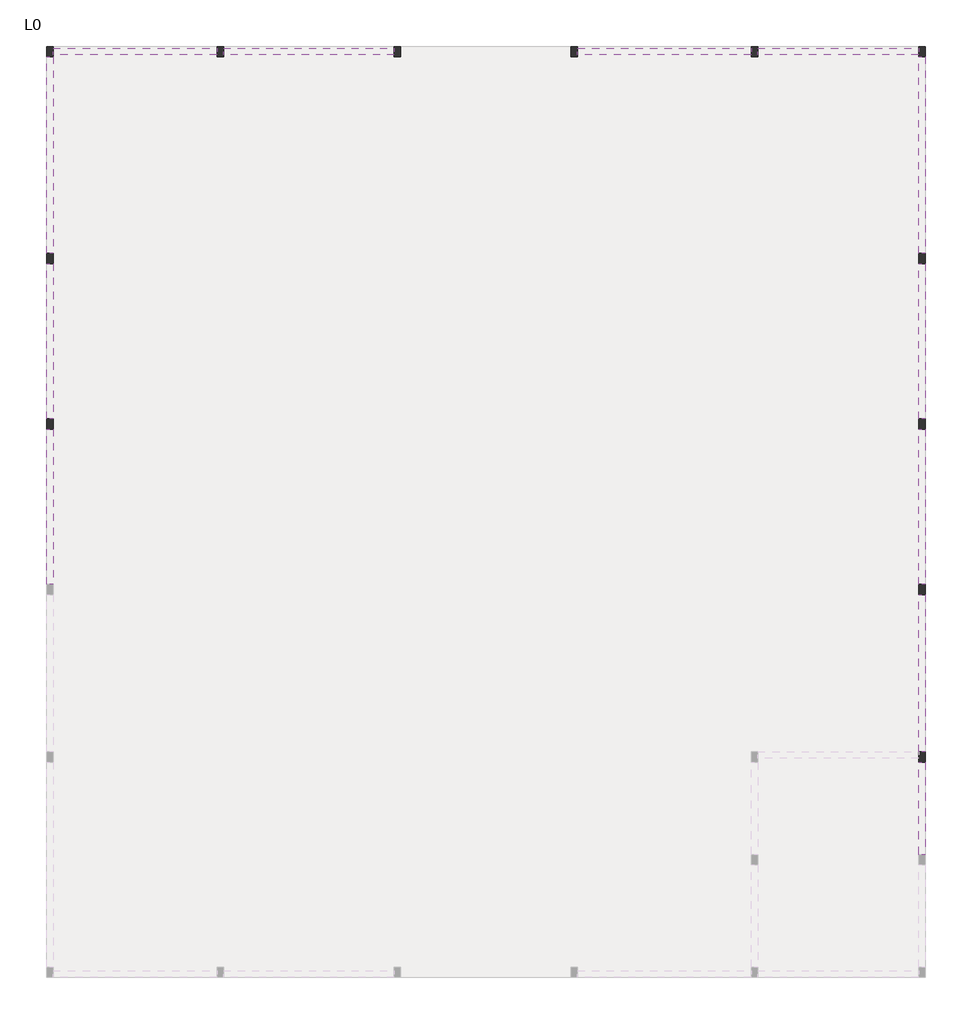
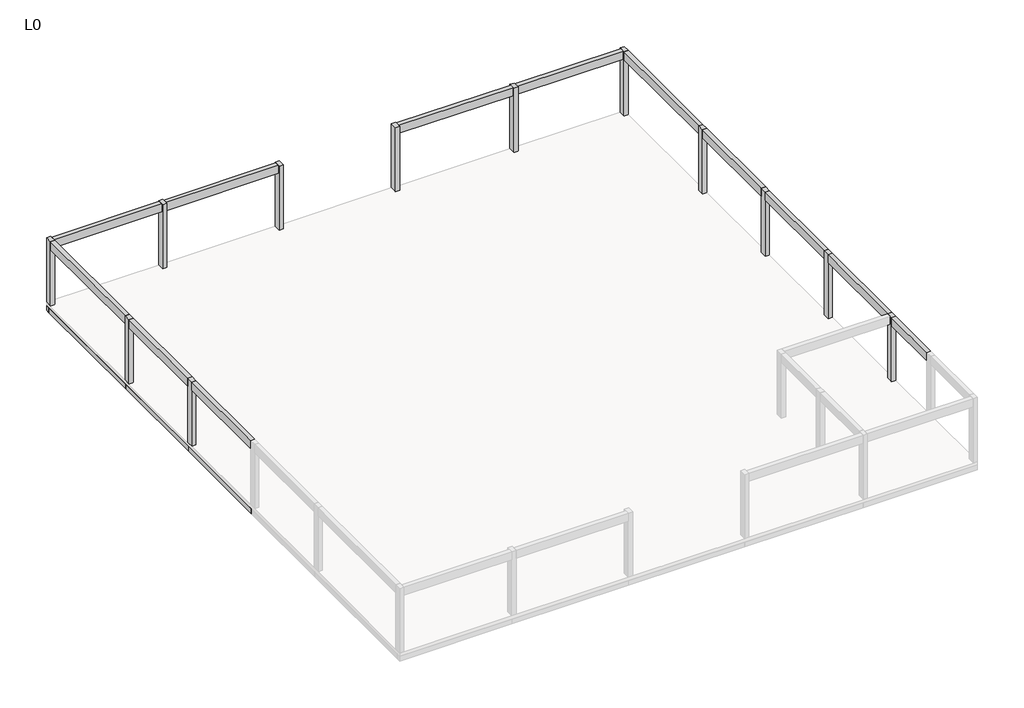
# One storey, part 2 of 2: 37 beams, 12 columns.
"""IFC4 building model written with IfcOpenShell, lengths in millimetres."""

import ifcopenshell
import ifcopenshell.guid

model = None  # the IFC model being written
_history = None  # IfcOwnerHistory: only IFC2X3 demands one
_inside = {}  # id of a spatial element -> (the spatial element, [elements in it])
_under = {}  # id of a project, library or spatial element -> (it, [spatial elements below it])
_declared = {}  # id of a project -> (the project, [libraries it declares])
_typed = {}  # id of a type object -> (the type object, [elements of that type])
_made_of = {}  # id of a material, layer set ... -> (it, [elements and type objects made of it])


def new_model(schema):
    """Start an empty IFC model of exactly this schema.

    Asked for "IFC4X3", IfcOpenShell would pick the latest addendum, in which some entities
    have other attributes; the version numbers below select the first issue.
    IFC2X3 requires an IfcOwnerHistory on every rooted entity: one is made here for all.
    """
    global model, _history
    if schema == "IFC4X3":
        model = ifcopenshell.file(schema_version=(4, 3, 0, 0))
    else:
        model = ifcopenshell.file(schema=schema)
    _inside.clear()
    _under.clear()
    _declared.clear()
    _typed.clear()
    _made_of.clear()
    _history = None
    if model.schema == "IFC2X3":
        org = make("IfcOrganization", Name="unknown")
        user = make(
            "IfcPersonAndOrganization",
            ThePerson=make("IfcPerson", FamilyName="unknown"),
            TheOrganization=org,
        )
        app = make(
            "IfcApplication",
            ApplicationDeveloper=org,
            Version="unknown",
            ApplicationFullName="unknown",
            ApplicationIdentifier="unknown",
        )
        _history = make(
            "IfcOwnerHistory",
            OwningUser=user,
            OwningApplication=app,
            ChangeAction="ADDED",
            CreationDate=0,
        )
    return model


def make(cls, **values):
    """One entity of the class cls with the attributes given. An attribute that is None is left unset."""
    return model.create_entity(
        cls, **{name: value for name, value in values.items() if value is not None}
    )


def rooted(cls, **values):
    """An entity with a GlobalId (a new one), such as an element, a storey or a relation."""
    return make(cls, GlobalId=ifcopenshell.guid.new(), OwnerHistory=_history, **values)


def si_unit(unit_type, name, prefix=None):
    """IfcSIUnit, for example si_unit("LENGTHUNIT", "METRE", prefix="MILLI")."""
    return make("IfcSIUnit", UnitType=unit_type, Prefix=prefix, Name=name)


def assignment(units):
    """IfcUnitAssignment: the units of a project."""
    return None if units is None else make("IfcUnitAssignment", Units=units)


def point(xyz):
    """IfcCartesianPoint."""
    return None if xyz is None else make("IfcCartesianPoint", Coordinates=xyz)


def direction(xyz):
    """IfcDirection."""
    return None if xyz is None else make("IfcDirection", DirectionRatios=xyz)


def frame(location, z_axis=None, x_axis=None):
    """IfcAxis2Placement3D, a coordinate frame: its origin and axes. An axis left out is left unset."""
    return make(
        "IfcAxis2Placement3D",
        Location=point(location),
        Axis=direction(z_axis),
        RefDirection=direction(x_axis),
    )


def origin():
    """The frame at (0, 0, 0) with its axes left unset."""
    return frame((0.0, 0.0, 0.0))


def origin_with_axes():
    """The frame at (0, 0, 0) with the z axis (0, 0, 1) and the x axis (1, 0, 0) written out."""
    return frame((0.0, 0.0, 0.0), z_axis=(0.0, 0.0, 1.0), x_axis=(1.0, 0.0, 0.0))


def place(relative_to, where):
    """IfcLocalPlacement: puts the frame where relative to a parent placement (None: the world)."""
    return make(
        "IfcLocalPlacement", PlacementRelTo=relative_to, RelativePlacement=where
    )


def context(
    kind, dimensions, precision=None, world=None, true_north=None, identifier=None
):
    """IfcGeometricRepresentationContext, for example the 3D "Model" context."""
    return make(
        "IfcGeometricRepresentationContext",
        ContextIdentifier=identifier,
        ContextType=kind,
        CoordinateSpaceDimension=dimensions,
        Precision=precision,
        WorldCoordinateSystem=world,
        TrueNorth=true_north,
    )


def project(units=None, contexts=None):
    """IfcProject with its units and contexts."""
    return rooted(
        "IfcProject",
        Name="project",
        RepresentationContexts=contexts,
        UnitsInContext=assignment(units),
    )


def spatial(cls, under=None, at=None, **own):
    """A site, building, storey or space (cls), placed at a placement, below another one or the project."""
    s = rooted(cls, ObjectPlacement=at, **own)
    if under is not None:
        _under.setdefault(under.id(), (under, []))[1].append(s)
    return s


def polyline(points):
    """IfcPolyline through the points."""
    return make("IfcPolyline", Points=[point(p) for p in points])


def outline(outer, holes=None, kind="AREA"):
    """IfcArbitraryClosedProfileDef: a profile drawn as a closed curve; with holes, ...WithVoids."""
    if holes is None:
        return make("IfcArbitraryClosedProfileDef", ProfileType=kind, OuterCurve=outer)
    return make(
        "IfcArbitraryProfileDefWithVoids",
        ProfileType=kind,
        OuterCurve=outer,
        InnerCurves=holes,
    )


def extrude(swept, where, along, depth):
    """IfcExtrudedAreaSolid: the profile swept, set in the frame where, extruded along a direction by depth."""
    return make(
        "IfcExtrudedAreaSolid",
        SweptArea=swept,
        Position=where,
        ExtrudedDirection=direction(along),
        Depth=depth,
    )


def faces_of(points, faces, orient=None, outer=None):
    """IfcFace entities. A face is a list of loops; a loop is a list of indices into points, from 0.

    orient and outer hold one flag for each loop. By default every Orientation is true, the
    first loop of a face is its IfcFaceOuterBound and the others are IfcFaceBound.
    """
    made = []
    for i, loops in enumerate(faces):
        bounds = []
        for j, loop in enumerate(loops):
            is_outer = j == 0 if outer is None else outer[i][j]
            bounds.append(
                make(
                    "IfcFaceOuterBound" if is_outer else "IfcFaceBound",
                    Bound=make("IfcPolyLoop", Polygon=[points[k] for k in loop]),
                    Orientation=True if orient is None else orient[i][j],
                )
            )
        made.append(make("IfcFace", Bounds=bounds))
    return made


def faceted_brep(points, faces, orient=None, outer=None, voids=None):
    """IfcFacetedBrep: a solid bounded by flat faces; with voids (closed shells), ...WithVoids."""
    shared = [point(p) for p in points]
    hull = make("IfcClosedShell", CfsFaces=faces_of(shared, faces, orient, outer))
    if voids is None:
        return make("IfcFacetedBrep", Outer=hull)
    return make(
        "IfcFacetedBrepWithVoids",
        Outer=hull,
        Voids=[
            make(cls, CfsFaces=faces_of(shared, fs, o, b)) for cls, fs, o, b in voids
        ],
    )


def shape(context_of_items, identifier, shape_type, items):
    """IfcShapeRepresentation: the items that make up one representation, for example the "Body"."""
    return make(
        "IfcShapeRepresentation",
        ContextOfItems=context_of_items,
        RepresentationIdentifier=identifier,
        RepresentationType=shape_type,
        Items=items,
    )


def made_of(thing, what):
    """Note that an element or type object is made of a material, layer set ...; save() writes the relation."""
    if what is not None:
        _made_of.setdefault(what.id(), (what, []))[1].append(thing)
    return thing


def element(
    cls,
    number,
    at=None,
    inside=None,
    cuts=None,
    type_object=None,
    material=None,
    context=None,
    identifier="Body",
    shape_type=None,
    held_by="IfcProductDefinitionShape",
    body=None,
    shapes=None,
    **own,
):
    """One element of the class cls, such as IfcWall. Its Tag is "e" and its number.

    at: its placement. inside: the storey or other place that contains it. cuts: it is an
    opening in that element (IfcRelVoidsElement). A single representation is given by context,
    identifier, shape_type and body (its items); several are given by shapes. held_by: the class
    of the entity that holds the representations. save() writes the other relations.
    """
    e = rooted(cls, Tag="e%d" % number, ObjectPlacement=at, **own)
    if body is not None:
        shapes = [shape(context, identifier, shape_type, body)]
    if shapes is not None:
        e.Representation = make(held_by, Representations=shapes)
    if inside is not None:
        _inside.setdefault(inside.id(), (inside, []))[1].append(e)
    if cuts is not None:
        rooted(
            "IfcRelVoidsElement", RelatingBuildingElement=cuts, RelatedOpeningElement=e
        )
    if type_object is not None:
        _typed.setdefault(type_object.id(), (type_object, []))[1].append(e)
    return made_of(e, material)


def aggregate(whole, parts):
    """IfcRelAggregates: a whole, such as a stair, and the parts it consists of."""
    return rooted("IfcRelAggregates", RelatingObject=whole, RelatedObjects=parts)


def save(model, path):
    """Write the relations noted so far, then the file.

    IfcRelAggregates (storeys below a building ...), IfcRelContainedInSpatialStructure (elements
    in a storey), IfcRelDefinesByType, IfcRelAssociatesMaterial and IfcRelDeclares: one each for
    every whole, place, type object, material and project.
    """
    for whole, parts in _under.values():
        aggregate(whole, parts)
    for where, things in _inside.values():
        rooted(
            "IfcRelContainedInSpatialStructure",
            RelatedElements=things,
            RelatingStructure=where,
        )
    for kind, things in _typed.values():
        rooted("IfcRelDefinesByType", RelatedObjects=things, RelatingType=kind)
    for what, things in _made_of.values():
        rooted("IfcRelAssociatesMaterial", RelatedObjects=things, RelatingMaterial=what)
    for by, libraries in _declared.values():
        rooted("IfcRelDeclares", RelatingContext=by, RelatedDefinitions=libraries)
    model.write(path)


model = new_model("IFC4")

# Units and contexts
model_context = context("Model", 3, world=origin())
ifc_project = project(units=[si_unit("LENGTHUNIT", "METRE", prefix="MILLI")], contexts=[model_context])

# Site, building, storey
site = spatial("IfcSite", under=ifc_project)
building = spatial("IfcBuilding", under=site)
storey = spatial("IfcBuildingStorey", under=building, Name="L0", Elevation=0.0)

# Beams
placement = place(None, origin())
element("IfcBeam", 1, ObjectType="Concrete-Rectangular Beam : 25 x 50", at=placement, inside=storey, context=model_context, shape_type="Brep", body=[
    faceted_brep([(17000.0, 18000.0, -500.0), (10270.0, 18000.0, -500.0), (10270.0, 18000.0, -200.0), (17000.0, 18000.0, -200.0), (10270.0, 17750.0, -500.0), (17000.0, 17750.0, -500.0), (16750.0, 17750.0, -500.0), (10520.0, 17750.0, -500.0), (17000.0, 17750.0, -200.0), (16750.0, 17750.0, -200.0), (10520.0, 17750.0, -200.0), (10270.0, 17750.0, -200.0)], [[[0, 1, 2, 3]], [[4, 1, 0, 5, 6, 7]], [[4, 7, 6, 5, 8, 9, 10, 11]], [[1, 4, 11, 2]], [[5, 0, 3, 8]], [[3, 2, 11, 10, 9, 8]]]),
])
element("IfcBeam", 2, ObjectType="Concrete-Rectangular Beam : 25 x 50", at=placement, inside=storey, context=model_context, shape_type="Brep", body=[
    faceted_brep([(10270.0, 18000.0, -500.0), (3300.0, 18000.0, -500.0), (3300.0, 18000.0, -200.0), (10270.0, 18000.0, -200.0), (3300.0, 17750.0, -500.0), (10270.0, 17750.0, -500.0), (3550.0, 17750.0, -500.0), (10270.0, 17750.0, -200.0), (3550.0, 17750.0, -200.0), (3300.0, 17750.0, -200.0)], [[[0, 1, 2, 3]], [[4, 1, 0, 5, 6]], [[4, 6, 5, 7, 8, 9]], [[1, 4, 9, 2]], [[5, 0, 3, 7]], [[3, 2, 9, 8, 7]]]),
])
element("IfcBeam", 3, ObjectType="Concrete-Rectangular Beam : 25 x 50", at=placement, inside=storey, context=model_context, shape_type="Brep", body=[
    faceted_brep([(3300.0, 18000.0, -500.0), (-3550.0, 18000.0, -500.0), (-3550.0, 18000.0, -200.0), (3300.0, 18000.0, -200.0), (-3550.0, 17750.0, -500.0), (3300.0, 17750.0, -500.0), (-3300.0, 17750.0, -500.0), (3300.0, 17750.0, -200.0), (-3300.0, 17750.0, -200.0), (-3550.0, 17750.0, -200.0)], [[[0, 1, 2, 3]], [[4, 1, 0, 5, 6]], [[4, 6, 5, 7, 8, 9]], [[1, 4, 9, 2]], [[5, 0, 3, 7]], [[3, 2, 9, 8, 7]]]),
])
element("IfcBeam", 4, ObjectType="Concrete-Rectangular Beam : 25 x 50", at=placement, inside=storey, context=model_context, shape_type="Brep", body=[
    faceted_brep([(-3550.0, 18000.0, -500.0), (-10400.0, 18000.0, -500.0), (-10400.0, 18000.0, -200.0), (-3550.0, 18000.0, -200.0), (-10400.0, 17750.0, -500.0), (-3550.0, 17750.0, -500.0), (-10150.0, 17750.0, -500.0), (-3550.0, 17750.0, -200.0), (-10150.0, 17750.0, -200.0), (-10400.0, 17750.0, -200.0)], [[[0, 1, 2, 3]], [[4, 1, 0, 5, 6]], [[4, 6, 5, 7, 8, 9]], [[1, 4, 9, 2]], [[5, 0, 3, 7]], [[3, 2, 9, 8, 7]]]),
])
element("IfcBeam", 5, ObjectType="Concrete-Rectangular Beam : 25 x 50", at=placement, inside=storey, context=model_context, shape_type="Brep", body=[
    faceted_brep([(-10400.0, 18000.0, -500.0), (-17000.0, 18000.0, -500.0), (-17000.0, 18000.0, -200.0), (-10400.0, 18000.0, -200.0), (-17000.0, 17750.0, -500.0), (-10400.0, 17750.0, -500.0), (-16750.0, 17750.0, -500.0), (-10400.0, 17750.0, -200.0), (-16750.0, 17750.0, -200.0), (-17000.0, 17750.0, -200.0)], [[[0, 1, 2, 3]], [[4, 1, 0, 5, 6]], [[4, 6, 5, 7, 8, 9]], [[1, 4, 9, 2]], [[5, 0, 3, 7]], [[3, 2, 9, 8, 7]]]),
])
element("IfcBeam", 6, ObjectType="Concrete-Rectangular Beam : 25 x 50", at=placement, inside=storey, context=model_context, shape_type="Brep", body=[
    faceted_brep([(17000.0, 9925.0, -500.0), (16750.0, 9925.0, -500.0), (10520.0, 9925.0, -500.0), (10520.0, 9925.0, -200.0), (16750.0, 9925.0, -200.0), (17000.0, 9925.0, -200.0), (17000.0, 9675.0, -500.0), (16750.0, 9675.0, -500.0), (10520.0, 9675.0, -500.0), (17000.0, 9675.0, -200.0), (16750.0, 9675.0, -200.0), (10520.0, 9675.0, -200.0)], [[[0, 1, 2, 3, 4, 5]], [[0, 6, 7, 8, 2, 1]], [[8, 7, 6, 9, 10, 11]], [[6, 0, 5, 9]], [[2, 8, 11, 3]], [[5, 4, 3, 11, 10, 9]]]),
])
element("IfcBeam", 7, ObjectType="Concrete-Rectangular Beam : 25 x 50", at=placement, inside=storey, context=model_context, shape_type="Brep", body=[
    faceted_brep([(17000.0, 3525.0, -500.0), (16750.0, 3525.0, -500.0), (10520.0, 3525.0, -500.0), (10270.0, 3525.0, -500.0), (3550.0, 3525.0, -500.0), (3300.0, 3525.0, -500.0), (-3300.0, 3525.0, -500.0), (-3550.0, 3525.0, -500.0), (-10150.0, 3525.0, -500.0), (-10150.0, 3525.0, -200.0), (-3550.0, 3525.0, -200.0), (-3300.0, 3525.0, -200.0), (3300.0, 3525.0, -200.0), (3550.0, 3525.0, -200.0), (10270.0, 3525.0, -200.0), (10520.0, 3525.0, -200.0), (16750.0, 3525.0, -200.0), (17000.0, 3525.0, -200.0), (17000.0, 3275.0, -500.0), (16750.0, 3275.0, -500.0), (10520.0, 3275.0, -500.0), (10270.0, 3275.0, -500.0), (3550.0, 3275.0, -500.0), (3300.0, 3275.0, -500.0), (-3300.0, 3275.0, -500.0), (-3550.0, 3275.0, -500.0), (-10150.0, 3275.0, -500.0), (17000.0, 3275.0, -200.0), (16750.0, 3275.0, -200.0), (10520.0, 3275.0, -200.0), (10270.0, 3275.0, -200.0), (3550.0, 3275.0, -200.0), (3300.0, 3275.0, -200.0), (-3300.0, 3275.0, -200.0), (-3550.0, 3275.0, -200.0), (-10150.0, 3275.0, -200.0)], [[[0, 1, 2, 3, 4, 5, 6, 7, 8, 9, 10, 11, 12, 13, 14, 15, 16, 17]], [[0, 18, 19, 20, 21, 22, 23, 24, 25, 26, 8, 7, 6, 5, 4, 3, 2, 1]], [[26, 25, 24, 23, 22, 21, 20, 19, 18, 27, 28, 29, 30, 31, 32, 33, 34, 35]], [[18, 0, 17, 27]], [[8, 26, 35, 9]], [[17, 16, 15, 14, 13, 12, 11, 10, 9, 35, 34, 33, 32, 31, 30, 29, 28, 27]]]),
])
element("IfcBeam", 8, ObjectType="Concrete-Rectangular Beam : 25 x 50", at=placement, inside=storey, context=model_context, shape_type="Brep", body=[
    faceted_brep([(-16750.0, -2875.0, -500.0), (-16750.0, 3275.0, -500.0), (-16750.0, 3525.0, -500.0), (-16750.0, 3525.0, -200.0), (-16750.0, 3275.0, -200.0), (-16750.0, -2875.0, -200.0), (-17000.0, 3525.0, -500.0), (-17000.0, -2875.0, -500.0), (-17000.0, -2875.0, -200.0), (-17000.0, 3525.0, -200.0)], [[[0, 1, 2, 3, 4, 5]], [[6, 2, 1, 0, 7]], [[6, 7, 8, 9]], [[2, 6, 9, 3]], [[7, 0, 5, 8]], [[5, 4, 3, 9, 8]]]),
])
element("IfcBeam", 9, ObjectType="Concrete-Rectangular Beam : 25 x 50", at=placement, inside=storey, context=model_context, shape_type="Brep", body=[
    faceted_brep([(-16750.0, 3525.0, -500.0), (-16750.0, 9675.0, -500.0), (-16750.0, 9925.0, -500.0), (-16750.0, 9925.0, -200.0), (-16750.0, 9675.0, -200.0), (-16750.0, 3525.0, -200.0), (-17000.0, 9925.0, -500.0), (-17000.0, 3525.0, -500.0), (-17000.0, 3525.0, -200.0), (-17000.0, 9925.0, -200.0)], [[[0, 1, 2, 3, 4, 5]], [[6, 2, 1, 0, 7]], [[6, 7, 8, 9]], [[2, 6, 9, 3]], [[7, 0, 5, 8]], [[5, 4, 3, 9, 8]]]),
])
element("IfcBeam", 10, ObjectType="Concrete-Rectangular Beam : 25 x 50", at=placement, inside=storey, context=model_context, shape_type="SweptSolid", body=[
    extrude(outline(polyline([(-17000.0, 17750.0), (-16750.0, 17750.0), (-16750.0, 9925.0), (-17000.0, 9925.0), (-17000.0, 17750.0)])), frame((0.0, 0.0, -500.0), z_axis=(0.0, 0.0, 1.0), x_axis=(1.0, 0.0, 0.0)), (0.0, 0.0, 1.0), 300.0),
])
element("IfcBeam", 11, ObjectType="Concrete-Rectangular Beam : 25 x 50", at=placement, inside=storey, context=model_context, shape_type="SweptSolid", body=[
    extrude(outline(polyline([(17000.0, -13448.5675387), (16750.0, -13448.5675387), (16750.0, -9595.0), (17000.0, -9595.0), (17000.0, -13448.5675387)])), frame((0.0, 0.0, -500.0), z_axis=(0.0, 0.0, 1.0), x_axis=(1.0, 0.0, 0.0)), (0.0, 0.0, 1.0), 300.0),
])
element("IfcBeam", 12, ObjectType="Concrete-Rectangular Beam : 25 x 50", at=placement, inside=storey, context=model_context, shape_type="SweptSolid", body=[
    extrude(outline(polyline([(16750.0, -3125.0), (17000.0, -3125.0), (17000.0, -9345.0), (16750.0, -9345.0), (16750.0, -3125.0)])), frame((0.0, 0.0, -500.0), z_axis=(0.0, 0.0, 1.0), x_axis=(1.0, 0.0, 0.0)), (0.0, 0.0, 1.0), 300.0),
])
element("IfcBeam", 13, ObjectType="Concrete-Rectangular Beam : 25 x 50", at=placement, inside=storey, context=model_context, shape_type="SweptSolid", body=[
    extrude(outline(polyline([(16750.0, 3275.0), (17000.0, 3275.0), (17000.0, -2875.0), (16750.0, -2875.0), (16750.0, 3275.0)])), frame((0.0, 0.0, -500.0), z_axis=(0.0, 0.0, 1.0), x_axis=(1.0, 0.0, 0.0)), (0.0, 0.0, 1.0), 300.0),
])
element("IfcBeam", 14, ObjectType="Concrete-Rectangular Beam : 25 x 50", at=placement, inside=storey, context=model_context, shape_type="SweptSolid", body=[
    extrude(outline(polyline([(16750.0, 9675.0), (17000.0, 9675.0), (17000.0, 3525.0), (16750.0, 3525.0), (16750.0, 9675.0)])), frame((0.0, 0.0, -500.0), z_axis=(0.0, 0.0, 1.0), x_axis=(1.0, 0.0, 0.0)), (0.0, 0.0, 1.0), 300.0),
])
element("IfcBeam", 15, ObjectType="Concrete-Rectangular Beam : 25 x 50", at=placement, inside=storey, context=model_context, shape_type="SweptSolid", body=[
    extrude(outline(polyline([(17000.0, 9925.0), (16750.0, 9925.0), (16750.0, 17750.0), (17000.0, 17750.0), (17000.0, 9925.0)])), frame((0.0, 0.0, -500.0), z_axis=(0.0, 0.0, 1.0), x_axis=(1.0, 0.0, 0.0)), (0.0, 0.0, 1.0), 300.0),
])
element("IfcBeam", 16, ObjectType="Concrete-Rectangular Beam : 25 x 50", at=placement, inside=storey, context=model_context, shape_type="SweptSolid", body=[
    extrude(outline(polyline([(-10400.0, 17750.0), (-10150.0, 17750.0), (-10150.0, 9925.0), (-10400.0, 9925.0), (-10400.0, 17750.0)])), frame((0.0, 0.0, -500.0), z_axis=(0.0, 0.0, 1.0), x_axis=(1.0, 0.0, 0.0)), (0.0, 0.0, 1.0), 300.0),
])
element("IfcBeam", 17, ObjectType="Concrete-Rectangular Beam : 25 x 50", at=placement, inside=storey, context=model_context, shape_type="SweptSolid", body=[
    extrude(outline(polyline([(-3550.0, 17750.0), (-3300.0, 17750.0), (-3300.0, 9925.0), (-3550.0, 9925.0), (-3550.0, 17750.0)])), frame((0.0, 0.0, -500.0), z_axis=(0.0, 0.0, 1.0), x_axis=(1.0, 0.0, 0.0)), (0.0, 0.0, 1.0), 300.0),
])
element("IfcBeam", 18, ObjectType="Concrete-Rectangular Beam : 25 x 50", at=placement, inside=storey, context=model_context, shape_type="SweptSolid", body=[
    extrude(outline(polyline([(3300.0, 17750.0), (3550.0, 17750.0), (3550.0, 9925.0), (3300.0, 9925.0), (3300.0, 17750.0)])), frame((0.0, 0.0, -500.0), z_axis=(0.0, 0.0, 1.0), x_axis=(1.0, 0.0, 0.0)), (0.0, 0.0, 1.0), 300.0),
])
element("IfcBeam", 19, ObjectType="Concrete-Rectangular Beam : 25 x 50", at=placement, inside=storey, context=model_context, shape_type="Brep", body=[
    faceted_brep([(10270.0, 9925.0, -500.0), (3550.0, 9925.0, -500.0), (3300.0, 9925.0, -500.0), (-3300.0, 9925.0, -500.0), (-3550.0, 9925.0, -500.0), (-10150.0, 9925.0, -500.0), (-10400.0, 9925.0, -500.0), (-16750.0, 9925.0, -500.0), (-16750.0, 9925.0, -200.0), (-10400.0, 9925.0, -200.0), (-10150.0, 9925.0, -200.0), (-3550.0, 9925.0, -200.0), (-3300.0, 9925.0, -200.0), (3300.0, 9925.0, -200.0), (3550.0, 9925.0, -200.0), (10270.0, 9925.0, -200.0), (-16750.0, 9675.0, -500.0), (10270.0, 9675.0, -500.0), (3550.0, 9675.0, -500.0), (3300.0, 9675.0, -500.0), (-3300.0, 9675.0, -500.0), (-3550.0, 9675.0, -500.0), (-10150.0, 9675.0, -500.0), (-10400.0, 9675.0, -500.0), (10270.0, 9675.0, -200.0), (3550.0, 9675.0, -200.0), (3300.0, 9675.0, -200.0), (-3300.0, 9675.0, -200.0), (-3550.0, 9675.0, -200.0), (-10150.0, 9675.0, -200.0), (-10400.0, 9675.0, -200.0), (-16750.0, 9675.0, -200.0)], [[[0, 1, 2, 3, 4, 5, 6, 7, 8, 9, 10, 11, 12, 13, 14, 15]], [[16, 7, 6, 5, 4, 3, 2, 1, 0, 17, 18, 19, 20, 21, 22, 23]], [[16, 23, 22, 21, 20, 19, 18, 17, 24, 25, 26, 27, 28, 29, 30, 31]], [[7, 16, 31, 8]], [[17, 0, 15, 24]], [[15, 14, 13, 12, 11, 10, 9, 8, 31, 30, 29, 28, 27, 26, 25, 24]]]),
])
element("IfcBeam", 20, ObjectType="Concrete-Rectangular Beam : 25 x 50", at=placement, inside=storey, context=model_context, shape_type="SweptSolid", body=[
    extrude(outline(polyline([(-16750.0, 3275.0), (-16750.0, 3525.0), (-10400.0, 3525.0), (-10400.0, 3275.0), (-16750.0, 3275.0)])), frame((0.0, 0.0, -500.0), z_axis=(0.0, 0.0, 1.0), x_axis=(1.0, 0.0, 0.0)), (0.0, 0.0, 1.0), 300.0),
])
element("IfcBeam", 21, ObjectType="Concrete-Rectangular Beam : 25 x 50", at=placement, inside=storey, context=model_context, shape_type="SweptSolid", body=[
    extrude(outline(polyline([(-3550.0, 9675.0), (-3300.0, 9675.0), (-3300.0, 3525.0), (-3550.0, 3525.0), (-3550.0, 9675.0)])), frame((0.0, 0.0, -500.0), z_axis=(0.0, 0.0, 1.0), x_axis=(1.0, 0.0, 0.0)), (0.0, 0.0, 1.0), 300.0),
])
element("IfcBeam", 22, ObjectType="Concrete-Rectangular Beam : 25 x 50", at=placement, inside=storey, context=model_context, shape_type="SweptSolid", body=[
    extrude(outline(polyline([(3300.0, 9675.0), (3550.0, 9675.0), (3550.0, 3525.0), (3300.0, 3525.0), (3300.0, 9675.0)])), frame((0.0, 0.0, -500.0), z_axis=(0.0, 0.0, 1.0), x_axis=(1.0, 0.0, 0.0)), (0.0, 0.0, 1.0), 300.0),
])
element("IfcBeam", 23, ObjectType="Concrete-Rectangular Beam : 25 x 50", at=placement, inside=storey, context=model_context, shape_type="Brep", body=[
    faceted_brep([(10520.0, 3525.0, -500.0), (10520.0, 9675.0, -500.0), (10520.0, 9925.0, -500.0), (10520.0, 17750.0, -500.0), (10520.0, 17750.0, -200.0), (10520.0, 9925.0, -200.0), (10520.0, 9675.0, -200.0), (10520.0, 3525.0, -200.0), (10270.0, 17750.0, -500.0), (10270.0, 3525.0, -500.0), (10270.0, 9675.0, -500.0), (10270.0, 9925.0, -500.0), (10270.0, 3525.0, -200.0), (10270.0, 9675.0, -200.0), (10270.0, 9925.0, -200.0), (10270.0, 17750.0, -200.0)], [[[0, 1, 2, 3, 4, 5, 6, 7]], [[8, 3, 2, 1, 0, 9, 10, 11]], [[8, 11, 10, 9, 12, 13, 14, 15]], [[3, 8, 15, 4]], [[9, 0, 7, 12]], [[7, 6, 5, 4, 15, 14, 13, 12]]]),
])
element("IfcBeam", 24, ObjectType="Concrete-Rectangular Beam : 25 x 50", at=placement, inside=storey, context=model_context, shape_type="SweptSolid", body=[
    extrude(outline(polyline([(3300.0, 3275.0), (3550.0, 3275.0), (3550.0, -2875.0), (3300.0, -2875.0), (3300.0, 3275.0)])), frame((0.0, 0.0, -500.0), z_axis=(0.0, 0.0, 1.0), x_axis=(1.0, 0.0, 0.0)), (0.0, 0.0, 1.0), 300.0),
])
element("IfcBeam", 25, ObjectType="Concrete-Rectangular Beam : 25 x 50", at=placement, inside=storey, context=model_context, shape_type="Brep", body=[
    faceted_brep([(-10150.0, -9345.0, -500.0), (-10150.0, -3125.0, -500.0), (-10150.0, -2875.0, -500.0), (-10150.0, 3275.0, -500.0), (-10150.0, 3525.0, -500.0), (-10150.0, 9675.0, -500.0), (-10150.0, 9675.0, -200.0), (-10150.0, 3525.0, -200.0), (-10150.0, 3275.0, -200.0), (-10150.0, -2875.0, -200.0), (-10150.0, -3125.0, -200.0), (-10150.0, -9345.0, -200.0), (-10400.0, 9675.0, -500.0), (-10400.0, -9345.0, -500.0), (-10400.0, -3125.0, -500.0), (-10400.0, -2875.0, -500.0), (-10400.0, 3275.0, -500.0), (-10400.0, 3525.0, -500.0), (-10400.0, -9345.0, -200.0), (-10400.0, -3125.0, -200.0), (-10400.0, -2875.0, -200.0), (-10400.0, 3275.0, -200.0), (-10400.0, 3525.0, -200.0), (-10400.0, 9675.0, -200.0)], [[[0, 1, 2, 3, 4, 5, 6, 7, 8, 9, 10, 11]], [[12, 5, 4, 3, 2, 1, 0, 13, 14, 15, 16, 17]], [[12, 17, 16, 15, 14, 13, 18, 19, 20, 21, 22, 23]], [[5, 12, 23, 6]], [[13, 0, 11, 18]], [[11, 10, 9, 8, 7, 6, 23, 22, 21, 20, 19, 18]]]),
])
element("IfcBeam", 26, ObjectType="Concrete-Rectangular Beam : 25 x 50", at=placement, inside=storey, context=model_context, shape_type="SweptSolid", body=[
    extrude(outline(polyline([(10520.0, 17675.0), (10520.0, 17925.0), (16750.0, 17925.0), (16750.0, 17675.0), (10520.0, 17675.0)])), frame((0.0, 0.0, 3500.0), z_axis=(0.0, 0.0, 1.0), x_axis=(1.0, 0.0, 0.0)), (0.0, 0.0, 1.0), 500.0),
])
element("IfcBeam", 27, ObjectType="Concrete-Rectangular Beam : 25 x 50", at=placement, inside=storey, context=model_context, shape_type="SweptSolid", body=[
    extrude(outline(polyline([(3550.0, 17675.0), (3550.0, 17925.0), (10270.0, 17925.0), (10270.0, 17675.0), (3550.0, 17675.0)])), frame((0.0, 0.0, 3500.0), z_axis=(0.0, 0.0, 1.0), x_axis=(1.0, 0.0, 0.0)), (0.0, 0.0, 1.0), 500.0),
])
element("IfcBeam", 28, ObjectType="Concrete-Rectangular Beam : 25 x 50", at=placement, inside=storey, context=model_context, shape_type="SweptSolid", body=[
    extrude(outline(polyline([(-10150.0, 17675.0), (-10150.0, 17925.0), (-3550.0, 17925.0), (-3550.0, 17675.0), (-10150.0, 17675.0)])), frame((0.0, 0.0, 3500.0), z_axis=(0.0, 0.0, 1.0), x_axis=(1.0, 0.0, 0.0)), (0.0, 0.0, 1.0), 500.0),
])
element("IfcBeam", 29, ObjectType="Concrete-Rectangular Beam : 25 x 50", at=placement, inside=storey, context=model_context, shape_type="SweptSolid", body=[
    extrude(outline(polyline([(-16750.0, 17675.0), (-16750.0, 17925.0), (-10400.0, 17925.0), (-10400.0, 17675.0), (-16750.0, 17675.0)])), frame((0.0, 0.0, 3500.0), z_axis=(0.0, 0.0, 1.0), x_axis=(1.0, 0.0, 0.0)), (0.0, 0.0, 1.0), 500.0),
])
element("IfcBeam", 30, ObjectType="Concrete-Rectangular Beam : 25 x 50", at=placement, inside=storey, context=model_context, shape_type="SweptSolid", body=[
    extrude(outline(polyline([(-17000.0, 3200.0), (-16750.0, 3200.0), (-16750.0, -2800.0), (-17000.0, -2800.0), (-17000.0, 3200.0)])), frame((0.0, 0.0, 3500.0), z_axis=(0.0, 0.0, 1.0), x_axis=(1.0, 0.0, 0.0)), (0.0, 0.0, 1.0), 500.0),
])
element("IfcBeam", 31, ObjectType="Concrete-Rectangular Beam : 25 x 50", at=placement, inside=storey, context=model_context, shape_type="SweptSolid", body=[
    extrude(outline(polyline([(-17000.0, 9600.0), (-16750.0, 9600.0), (-16750.0, 3600.0), (-17000.0, 3600.0), (-17000.0, 9600.0)])), frame((0.0, 0.0, 3500.0), z_axis=(0.0, 0.0, 1.0), x_axis=(1.0, 0.0, 0.0)), (0.0, 0.0, 1.0), 500.0),
])
element("IfcBeam", 32, ObjectType="Concrete-Rectangular Beam : 25 x 50", at=placement, inside=storey, context=model_context, shape_type="SweptSolid", body=[
    extrude(outline(polyline([(-17000.0, 17600.0), (-16750.0, 17600.0), (-16750.0, 10000.0), (-17000.0, 10000.0), (-17000.0, 17600.0)])), frame((0.0, 0.0, 3500.0), z_axis=(0.0, 0.0, 1.0), x_axis=(1.0, 0.0, 0.0)), (0.0, 0.0, 1.0), 500.0),
])
element("IfcBeam", 33, ObjectType="Concrete-Rectangular Beam : 25 x 50", at=placement, inside=storey, context=model_context, shape_type="SweptSolid", body=[
    extrude(outline(polyline([(16750.0, -9670.0), (17000.0, -9670.0), (17000.0, -13248.5675387), (16750.0, -13248.5675387), (16750.0, -9670.0)])), frame((0.0, 0.0, 3500.0), z_axis=(0.0, 0.0, 1.0), x_axis=(1.0, 0.0, 0.0)), (0.0, 0.0, 1.0), 500.0),
])
element("IfcBeam", 34, ObjectType="Concrete-Rectangular Beam : 25 x 50", at=placement, inside=storey, context=model_context, shape_type="SweptSolid", body=[
    extrude(outline(polyline([(16750.0, -3200.0), (17000.0, -3200.0), (17000.0, -9270.0), (16750.0, -9270.0), (16750.0, -3200.0)])), frame((0.0, 0.0, 3500.0), z_axis=(0.0, 0.0, 1.0), x_axis=(1.0, 0.0, 0.0)), (0.0, 0.0, 1.0), 500.0),
])
element("IfcBeam", 35, ObjectType="Concrete-Rectangular Beam : 25 x 50", at=placement, inside=storey, context=model_context, shape_type="SweptSolid", body=[
    extrude(outline(polyline([(16750.0, 3200.0), (17000.0, 3200.0), (17000.0, -2800.0), (16750.0, -2800.0), (16750.0, 3200.0)])), frame((0.0, 0.0, 3500.0), z_axis=(0.0, 0.0, 1.0), x_axis=(1.0, 0.0, 0.0)), (0.0, 0.0, 1.0), 500.0),
])
element("IfcBeam", 36, ObjectType="Concrete-Rectangular Beam : 25 x 50", at=placement, inside=storey, context=model_context, shape_type="SweptSolid", body=[
    extrude(outline(polyline([(16750.0, 9600.0), (17000.0, 9600.0), (17000.0, 3600.0), (16750.0, 3600.0), (16750.0, 9600.0)])), frame((0.0, 0.0, 3500.0), z_axis=(0.0, 0.0, 1.0), x_axis=(1.0, 0.0, 0.0)), (0.0, 0.0, 1.0), 500.0),
])
element("IfcBeam", 37, ObjectType="Concrete-Rectangular Beam : 25 x 50", at=placement, inside=storey, context=model_context, shape_type="SweptSolid", body=[
    extrude(outline(polyline([(16750.0, 17600.0), (17000.0, 17600.0), (17000.0, 10000.0), (16750.0, 10000.0), (16750.0, 17600.0)])), frame((0.0, 0.0, 3500.0), z_axis=(0.0, 0.0, 1.0), x_axis=(1.0, 0.0, 0.0)), (0.0, 0.0, 1.0), 500.0),
])

# Columns
element("IfcColumn", 38, ObjectType="M_Concrete-Rectangular-Column : 250 x 400mm", at=placement, inside=storey, context=model_context, shape_type="SweptSolid", body=[
    extrude(outline(polyline([(-17000.0, 17600.0), (-17000.0, 18000.0), (-16750.0, 18000.0), (-16750.0, 17600.0), (-17000.0, 17600.0)])), origin_with_axes(), (0.0, 0.0, 1.0), 4000.0),
])
element("IfcColumn", 39, ObjectType="M_Concrete-Rectangular-Column : 250 x 400mm", at=placement, inside=storey, context=model_context, shape_type="SweptSolid", body=[
    extrude(outline(polyline([(-10400.0, 17600.0), (-10400.0, 18000.0), (-10150.0, 18000.0), (-10150.0, 17600.0), (-10400.0, 17600.0)])), origin_with_axes(), (0.0, 0.0, 1.0), 4000.0),
])
element("IfcColumn", 40, ObjectType="M_Concrete-Rectangular-Column : 250 x 400mm", at=placement, inside=storey, context=model_context, shape_type="SweptSolid", body=[
    extrude(outline(polyline([(-3550.0, 17600.0), (-3550.0, 18000.0), (-3300.0, 18000.0), (-3300.0, 17600.0), (-3550.0, 17600.0)])), origin_with_axes(), (0.0, 0.0, 1.0), 4000.0),
])
element("IfcColumn", 41, ObjectType="M_Concrete-Rectangular-Column : 250 x 400mm", at=placement, inside=storey, context=model_context, shape_type="SweptSolid", body=[
    extrude(outline(polyline([(3300.0, 17600.0), (3300.0, 18000.0), (3550.0, 18000.0), (3550.0, 17600.0), (3300.0, 17600.0)])), origin_with_axes(), (0.0, 0.0, 1.0), 4000.0),
])
element("IfcColumn", 42, ObjectType="M_Concrete-Rectangular-Column : 250 x 400mm", at=placement, inside=storey, context=model_context, shape_type="SweptSolid", body=[
    extrude(outline(polyline([(10270.0, 17600.0), (10270.0, 18000.0), (10520.0, 18000.0), (10520.0, 17600.0), (10270.0, 17600.0)])), origin_with_axes(), (0.0, 0.0, 1.0), 4000.0),
])
element("IfcColumn", 43, ObjectType="M_Concrete-Rectangular-Column : 250 x 400mm", at=placement, inside=storey, context=model_context, shape_type="SweptSolid", body=[
    extrude(outline(polyline([(16750.0, 17600.0), (16750.0, 18000.0), (17000.0, 18000.0), (17000.0, 17600.0), (16750.0, 17600.0)])), origin_with_axes(), (0.0, 0.0, 1.0), 4000.0),
])
element("IfcColumn", 44, ObjectType="M_Concrete-Rectangular-Column : 250 x 400mm", at=placement, inside=storey, context=model_context, shape_type="SweptSolid", body=[
    extrude(outline(polyline([(-17000.0, 9600.0), (-17000.0, 10000.0), (-16750.0, 10000.0), (-16750.0, 9600.0), (-17000.0, 9600.0)])), origin_with_axes(), (0.0, 0.0, 1.0), 4000.0),
])
element("IfcColumn", 45, ObjectType="M_Concrete-Rectangular-Column : 250 x 400mm", at=placement, inside=storey, context=model_context, shape_type="SweptSolid", body=[
    extrude(outline(polyline([(16750.0, 9600.0), (16750.0, 10000.0), (17000.0, 10000.0), (17000.0, 9600.0), (16750.0, 9600.0)])), origin_with_axes(), (0.0, 0.0, 1.0), 4000.0),
])
element("IfcColumn", 46, ObjectType="M_Concrete-Rectangular-Column : 250 x 400mm", at=placement, inside=storey, context=model_context, shape_type="SweptSolid", body=[
    extrude(outline(polyline([(-17000.0, 3200.0), (-17000.0, 3600.0), (-16750.0, 3600.0), (-16750.0, 3200.0), (-17000.0, 3200.0)])), origin_with_axes(), (0.0, 0.0, 1.0), 4000.0),
])
element("IfcColumn", 47, ObjectType="M_Concrete-Rectangular-Column : 250 x 400mm", at=placement, inside=storey, context=model_context, shape_type="SweptSolid", body=[
    extrude(outline(polyline([(16750.0, 3200.0), (16750.0, 3600.0), (17000.0, 3600.0), (17000.0, 3200.0), (16750.0, 3200.0)])), origin_with_axes(), (0.0, 0.0, 1.0), 4000.0),
])
element("IfcColumn", 48, ObjectType="M_Concrete-Rectangular-Column : 250 x 400mm", at=placement, inside=storey, context=model_context, shape_type="SweptSolid", body=[
    extrude(outline(polyline([(16750.0, -3200.0), (16750.0, -2800.0), (17000.0, -2800.0), (17000.0, -3200.0), (16750.0, -3200.0)])), origin_with_axes(), (0.0, 0.0, 1.0), 4000.0),
])
element("IfcColumn", 49, ObjectType="M_Concrete-Rectangular-Column : 250 x 400mm", at=placement, inside=storey, context=model_context, shape_type="SweptSolid", body=[
    extrude(outline(polyline([(16750.0, -9670.0), (16750.0, -9270.0), (17000.0, -9270.0), (17000.0, -9670.0), (16750.0, -9670.0)])), origin_with_axes(), (0.0, 0.0, 1.0), 4000.0),
])

save(model, "model.ifc")

# Revit data of these elements
# Type "Concrete-Rectangular Beam : 25 x 50"
#   Length [instance default] = 1.524 m
#   b = 0.25 m
#   h = 0.50 m
#   Structural Material [instance default] = Concrete, Cast-in-Place gray
#   Assembly Code = ""
# Type "M_Concrete-Rectangular-Column : 250 x 400mm"
#   b = 0.25 m
#   h = 0.40 m
#   Structural Material [instance default] = Concrete, Cast-in-Place gray
# Elements 1, 6, 26 (IfcBeam, "Concrete-Rectangular Beam : 25 x 50")
#   Length = 6.48 m
#   Structural Material = Concrete, Cast-in-Place gray
#   Phase Created = New Construction
#   Materials on its faces: "Concrete, Cast-in-Place gray"
# Elements 2, 27 (IfcBeam, "Concrete-Rectangular Beam : 25 x 50")
#   Length = 6.97 m
#   Structural Material = Concrete, Cast-in-Place gray
#   Phase Created = New Construction
#   Materials on its faces: "Concrete, Cast-in-Place gray"
# Elements 3, 4, 28 (IfcBeam, "Concrete-Rectangular Beam : 25 x 50")
#   Length = 6.85 m
#   Structural Material = Concrete, Cast-in-Place gray
#   Phase Created = New Construction
#   Materials on its faces: "Concrete, Cast-in-Place gray"
# Elements 5, 29 (IfcBeam, "Concrete-Rectangular Beam : 25 x 50")
#   Length = 6.60 m
#   Structural Material = Concrete, Cast-in-Place gray
#   Phase Created = New Construction
#   Materials on its faces: "Concrete, Cast-in-Place gray"
# Element 7 (IfcBeam, "Concrete-Rectangular Beam : 25 x 50")
#   Length = 27.15 m
#   Structural Material = Concrete, Cast-in-Place gray
#   Phase Created = New Construction
#   Materials on its faces: "Concrete, Cast-in-Place gray"
# Elements 8, 9, 13, 14, 30, 31, 35, 36 (IfcBeam, "Concrete-Rectangular Beam : 25 x 50")
#   Length = 6.40 m
#   Structural Material = Concrete, Cast-in-Place gray
#   Phase Created = New Construction
#   Materials on its faces: "Concrete, Cast-in-Place gray"
# Elements 10, 15 (IfcBeam, "Concrete-Rectangular Beam : 25 x 50")
#   Length = 8.075 m
#   Structural Material = Concrete, Cast-in-Place gray
#   Phase Created = New Construction
#   Materials on its faces: "Concrete, Cast-in-Place gray"
# Elements 11, 33 (IfcBeam, "Concrete-Rectangular Beam : 25 x 50")
#   Length = 3.978568 m
#   Structural Material = Concrete, Cast-in-Place gray
#   Phase Created = New Construction
#   Materials on its faces: "Concrete, Cast-in-Place gray"
# Elements 12, 34 (IfcBeam, "Concrete-Rectangular Beam : 25 x 50")
#   Length = 6.47 m
#   Structural Material = Concrete, Cast-in-Place gray
#   Phase Created = New Construction
#   Materials on its faces: "Concrete, Cast-in-Place gray"
# Elements 16, 25 (IfcBeam, "Concrete-Rectangular Beam : 25 x 50")
#   IfcGUID = "2BzmfI2393bxdTxu7BJEPq"
#   Phase Created = New Construction
#   Materials on its faces: "Concrete, Cast-in-Place gray"
# Elements 17, 21 (IfcBeam, "Concrete-Rectangular Beam : 25 x 50")
#   IfcGUID = "2BzmfI2393bxdTxu7BJEPw"
#   Phase Created = New Construction
#   Materials on its faces: "Concrete, Cast-in-Place gray"
# Elements 18, 22, 24 (IfcBeam, "Concrete-Rectangular Beam : 25 x 50")
#   IfcGUID = "2BzmfI2393bxdTxu7BJEPx"
#   Phase Created = New Construction
#   Materials on its faces: "Concrete, Cast-in-Place gray"
# Element 19 (IfcBeam, "Concrete-Rectangular Beam : 25 x 50")
#   IfcGUID = "2BzmfI2393bxdTxu7BJEPZ"
#   Phase Created = New Construction
#   Materials on its faces: "Concrete, Cast-in-Place gray"
# Element 20 (IfcBeam, "Concrete-Rectangular Beam : 25 x 50")
#   IfcGUID = "2BzmfI2393bxdTxu7BJEPX"
#   Phase Created = New Construction
#   Materials on its faces: "Concrete, Cast-in-Place gray"
# Element 23 (IfcBeam, "Concrete-Rectangular Beam : 25 x 50")
#   IfcGUID = "2BzmfI2393bxdTxu7BJEPy"
#   Phase Created = New Construction
#   Materials on its faces: "Concrete, Cast-in-Place gray"
# Elements 32, 37 (IfcBeam, "Concrete-Rectangular Beam : 25 x 50")
#   Length = 8.00 m
#   Structural Material = Concrete, Cast-in-Place gray
#   Phase Created = New Construction
#   Materials on its faces: "Concrete, Cast-in-Place gray"
# Elements 38, 39, 40, 41, 42, 43, 44, 45, 46, 47, 48, 49 (IfcColumn, "M_Concrete-Rectangular-Column : 250 x 400mm")
#   Structural Material = Concrete, Cast-in-Place gray
#   Phase Created = New Construction
#   Materials on its faces: "Concrete, Cast-in-Place gray"
# Materials
#   "Concrete, Cast-in-Place gray": class "Concrete", colour RGB 192 192 192, transparency 0, Description = "Cast-in-place concrete", Cost = 0
